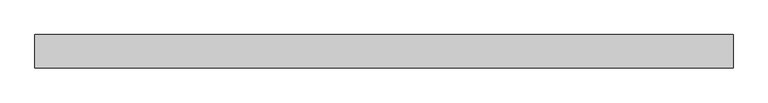
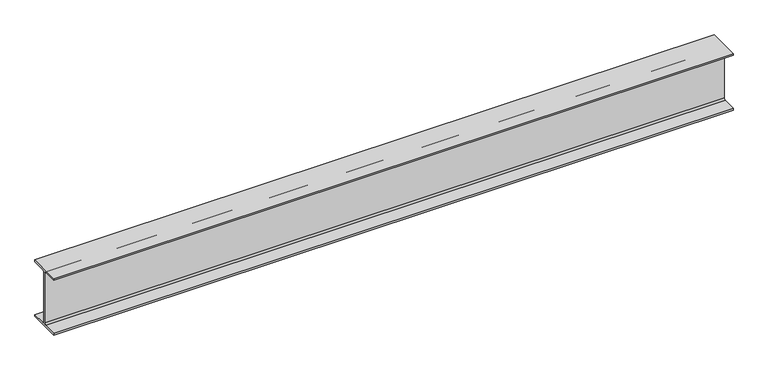
"""IFC4 building model written with IfcOpenShell, lengths in millimetres: beam geometry, Old_Steel Beam_H-KSD3502 : H_SB_ASB_H-200×200x8x12."""

from ifc_helpers import new_model, si_unit, point, frame, frame_2d, origin, place, context, project, spatial, polyline, circle_curve, trimmed, segment, composite_curve, outline, extrude, source, transform, mapped, element, save


def beam_b71a2e39(model_context):
    return source(origin(), model_context, "Body", "SweptSolid", [
        extrude(outline(composite_curve([segment(polyline([(82.5, -141.5), (82.5, -151.7), (-82.5, -151.7), (-82.5, -141.5), (-11.9, -141.5)]), True, "CONTINUOUS"), segment(trimmed(circle_curve(frame_2d((-11.9, -132.6)), 8.9), [point((-11.9, -141.5))], [point((-3.0, -132.6))], True, "CARTESIAN"), True, "CONTINUOUS"), segment(polyline([(-3.0, -132.6), (-3.0, 132.6)]), True, "CONTINUOUS"), segment(trimmed(circle_curve(frame_2d((-11.9, 132.6)), 8.9), [point((-3.0, 132.6))], [point((-11.9, 141.5))], True, "CARTESIAN"), True, "CONTINUOUS"), segment(polyline([(-11.9, 141.5), (-82.5, 141.5), (-82.5, 151.7), (82.5, 151.7), (82.5, 141.5), (11.9, 141.5)]), True, "CONTINUOUS"), segment(trimmed(circle_curve(frame_2d((11.9, 132.6)), 8.9), [point((11.9, 141.5))], [point((3.0, 132.6))], True, "CARTESIAN"), True, "CONTINUOUS"), segment(polyline([(3.0, 132.6), (3.0, -132.6)]), True, "CONTINUOUS"), segment(trimmed(circle_curve(frame_2d((11.9, -132.6)), 8.9), [point((3.0, -132.6))], [point((11.9, -141.5))], True, "CARTESIAN"), True, "CONTINUOUS"), segment(polyline([(11.9, -141.5), (82.5, -141.5)]), True, "CONTINUOUS")], self_intersect=False)), frame((-1683.7594404, 0.0, 0.0), z_axis=(1.0, 0.0, 0.0), x_axis=(0.0, 1.0, 0.0)), (0.0, 0.0, 1.0), 3450.380526),
    ])


if __name__ == "__main__":
    model = new_model("IFC4")
    model_context = context("Model", 3, world=origin())
    ifc_project = project(units=[si_unit("LENGTHUNIT", "METRE", prefix="MILLI")], contexts=[model_context])
    site = spatial("IfcSite", under=ifc_project)
    building = spatial("IfcBuilding", under=site)
    placement = place(None, origin())
    beam_shape = beam_b71a2e39(model_context)
    element("IfcBeam", 1, ObjectType="Old_Steel Beam_H-KSD3502 : H_SB_ASB_H-200×200x8x12", at=placement, inside=building, context=model_context, shape_type="MappedRepresentation", body=[
        mapped(beam_shape, transform((0.0, 0.0, 0.0), x_axis=(1.0, 0.0, 0.0), y_axis=(0.0, 1.0, 0.0), z_axis=(0.0, 0.0, 1.0))),
    ])
    save(model, "model.ifc")

# Revit data of these elements
# Type "Old_Steel Beam_H-KSD3502 : H_SB_ASB_H-200×200x8x12"
#   Width = 20.0 cm
#   Web Thickness = 0.8 cm
#   Web Fillet = 1.3 cm
#   Warping Constant = 141376.0 cm⁶
#   Torsional Moment of Inertia = 26.2485 cm⁴
#   Torsional Modulus = 1.0 cm³
#   Section Area = 63.53 cm²
#   Plastic Modulus weak axis = 244.0 cm³
#   Plastic Modulus strong axis = 525.0 cm³
#   Perimeter = 1.16 m²/m
#   Nominal Weight = 49.90 kgf/m
#   Moment of Inertia weak axis = 1600.00 cm⁴
#   Moment of Inertia strong axis = 4720.00 cm⁴
#   Height = 20.0 cm
#   Flange Thickness = 1.2 cm
#   Elastic Modulus weak axis = 160.0 cm³
#   Elastic Modulus strong axis = 472.0 cm³
#   Centroid Vertical = 10.0 cm
#   Centroid Horizontal = 10.0 cm
#   Length [instance default] = 1.5240 m
#   Structural Material [instance default] = Steel, 45-345
#   Assembly Code = ""
# Element 1 (IfcBeam, "Old_Steel Beam_H-KSD3502 : H_SB_ASB_H-200×200x8x12")
#   Structural Material = none
# Materials
#   "Steel, 45-345": class "Metal", colour RGB 189 187 185, transparency 0, Description = "Steel 345 MPa", Cost = 0
